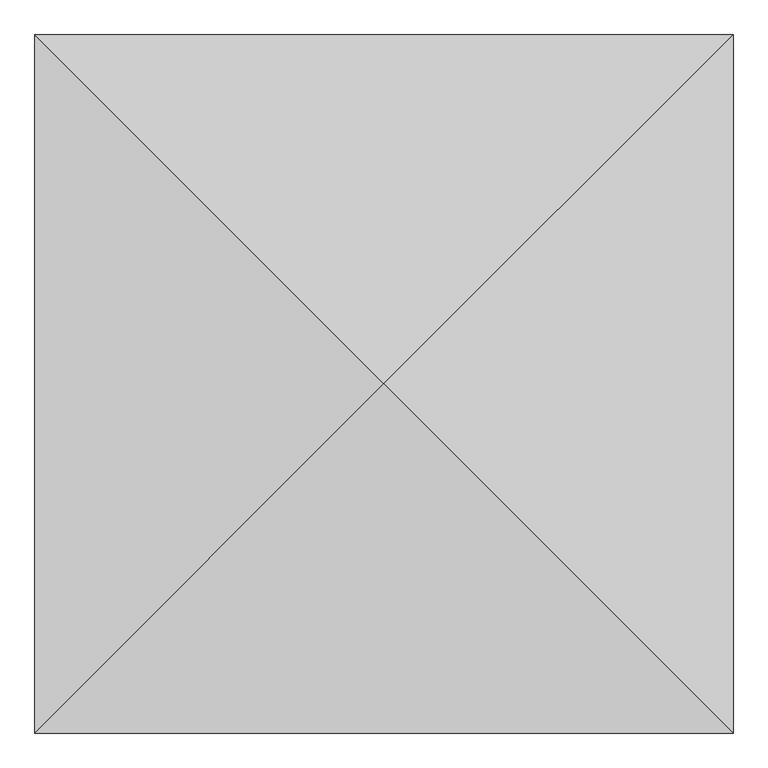
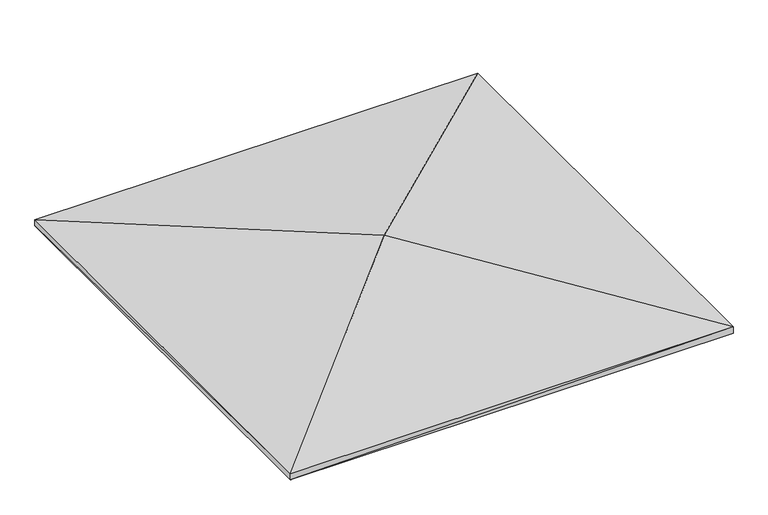
"""IFC4 building model written with IfcOpenShell, lengths in millimetres: geographic element geometry, Enscape AssetDefinition - Stone 002 Pebbles : Enscape AssetDefinition - Stone 002 Pebbles."""

from ifc_helpers import new_model, si_unit, origin, place, context, project, spatial, faceted_brep, source, transform, mapped, element, save


def geographic_element_ffb6b139(model_context):
    return source(origin(), model_context, "Body", "Brep", [
        faceted_brep([(999.1142154, 999.1142154, 0.0), (-999.1142154, -999.1142154, 0.0), (-999.1142154, 999.1142154, 0.0), (999.1142154, -999.1142154, 0.0), (999.1142154, -999.1142154, 29.9493484), (-999.1142154, -999.1142154, 29.9493484), (999.1142154, 999.1142154, 29.9493428), (-999.1142154, 999.1142154, 29.9493428), (0.0, -1.9e-06, 212.2415751)], [[[0, 1, 2]], [[1, 0, 3]], [[4, 1, 3]], [[1, 4, 5]], [[6, 3, 0]], [[3, 6, 4]], [[7, 0, 2]], [[0, 7, 6]], [[5, 2, 1]], [[2, 5, 7]], [[8, 5, 4]], [[8, 4, 6]], [[8, 6, 7]], [[8, 7, 5]]]),
    ])


if __name__ == "__main__":
    model = new_model("IFC4")
    model_context = context("Model", 3, world=origin())
    ifc_project = project(units=[si_unit("LENGTHUNIT", "METRE", prefix="MILLI")], contexts=[model_context])
    site = spatial("IfcSite", under=ifc_project)
    building = spatial("IfcBuilding", under=site)
    placement = place(None, origin())
    geographic_element_shape = geographic_element_ffb6b139(model_context)
    element("IfcGeographicElement", 1, ObjectType="Enscape AssetDefinition - Stone 002 Pebbles : Enscape AssetDefinition - Stone 002 Pebbles", at=placement, inside=building, context=model_context, shape_type="MappedRepresentation", body=[
        mapped(geographic_element_shape, transform((0.0, 0.0, 0.0), x_axis=(1.0, 0.0, 0.0), y_axis=(0.0, 1.0, 0.0), z_axis=(0.0, 0.0, 1.0))),
    ])
    save(model, "model.ifc")

# Revit data of these elements
# Type "Enscape AssetDefinition - Stone 002 Pebbles : Enscape AssetDefinition - Stone 002 Pebbles"
#   EnscapeAssetSource = "REMOTE"
#   EnscapeAssetId = "04fc6e15-b291-4b78-af55-c23c3feeb414"
#   Height = 0.212242 m
#   EnscapeNativeAssetHeight = 0.212242 m
#   Default Elevation = 0
